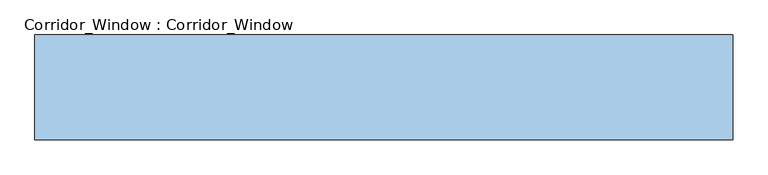
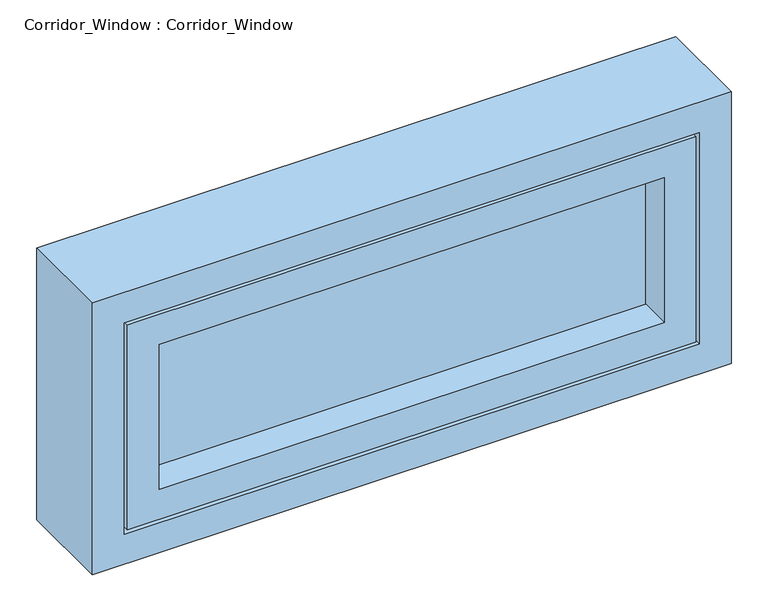
"""IFC4 building model written with IfcOpenShell, lengths in millimetres: window geometry, Corridor_Window : Corridor_Window."""

from ifc_helpers import new_model, si_unit, frame, origin, place, context, project, spatial, polyline, outline, extrude, source, transform, mapped, element, save


def corridor_window_corridor_window_b9059d84(model_context):
    return source(origin(), model_context, "Body", "SweptSolid", [
        extrude(outline(polyline([(1035.0, 405.0), (1825.0, 405.0), (1825.0, 395.0), (1035.0, 395.0), (1035.0, 405.0)])), frame((0.0, 0.0, 2105.0), z_axis=(0.0, 0.0, 1.0), x_axis=(1.0, 0.0, 0.0)), (0.0, 0.0, 1.0), 240.0),
        extrude(outline(polyline([(2055.0, 1875.0), (2395.0, 1875.0), (2395.0, 985.0), (2055.0, 985.0), (2055.0, 1875.0)]), holes=[polyline([(2105.0, 1035.0), (2345.0, 1035.0), (2345.0, 1825.0), (2105.0, 1825.0), (2105.0, 1035.0)])]), frame((0.0, 345.0, 0.0), z_axis=(0.0, 1.0, 0.0), x_axis=(0.0, 0.0, 1.0)), (0.0, 0.0, 1.0), 100.0),
        extrude(outline(polyline([(2000.0, 1930.0), (2450.0, 1930.0), (2450.0, 930.0), (2000.0, 930.0), (2000.0, 1930.0)]), holes=[polyline([(2050.0, 980.0), (2400.0, 980.0), (2400.0, 1880.0), (2050.0, 1880.0), (2050.0, 980.0)])]), frame((0.0, 345.0, 0.0), z_axis=(0.0, 1.0, 0.0), x_axis=(0.0, 0.0, 1.0)), (0.0, 0.0, 1.0), 150.0),
    ])


if __name__ == "__main__":
    model = new_model("IFC4")
    model_context = context("Model", 3, world=origin())
    ifc_project = project(units=[si_unit("LENGTHUNIT", "METRE", prefix="MILLI")], contexts=[model_context])
    site = spatial("IfcSite", under=ifc_project)
    building = spatial("IfcBuilding", under=site)
    placement = place(None, origin())
    corridor_window_corridor_window_shape = corridor_window_corridor_window_b9059d84(model_context)
    element("IfcWindow", 1, ObjectType="Corridor_Window : Corridor_Window", at=placement, inside=building, context=model_context, shape_type="MappedRepresentation", body=[
        mapped(corridor_window_corridor_window_shape, transform((0.0, 0.0, 0.0), x_axis=(1.0, 0.0, 0.0), y_axis=(0.0, 1.0, 0.0), z_axis=(0.0, 0.0, 1.0))),
    ])
    save(model, "model.ifc")

# Revit data of these elements
# Type "Corridor_Window : Corridor_Window"
#   Type Mark = "55"
#   NameOverride = "Corridor_Window"
# Element 1 (IfcWindow, "Corridor_Window : Corridor_Window")
#   Materials on its faces: "IfcSurfaceStyle #392", "IfcSurfaceStyle #398"
# Materials
#   "IfcSurfaceStyle #392": class "Unassigned", colour RGB 204 204 204, transparency 0
#   "IfcSurfaceStyle #398": class "Unassigned", colour RGB 93 183 203, transparency 0.85
